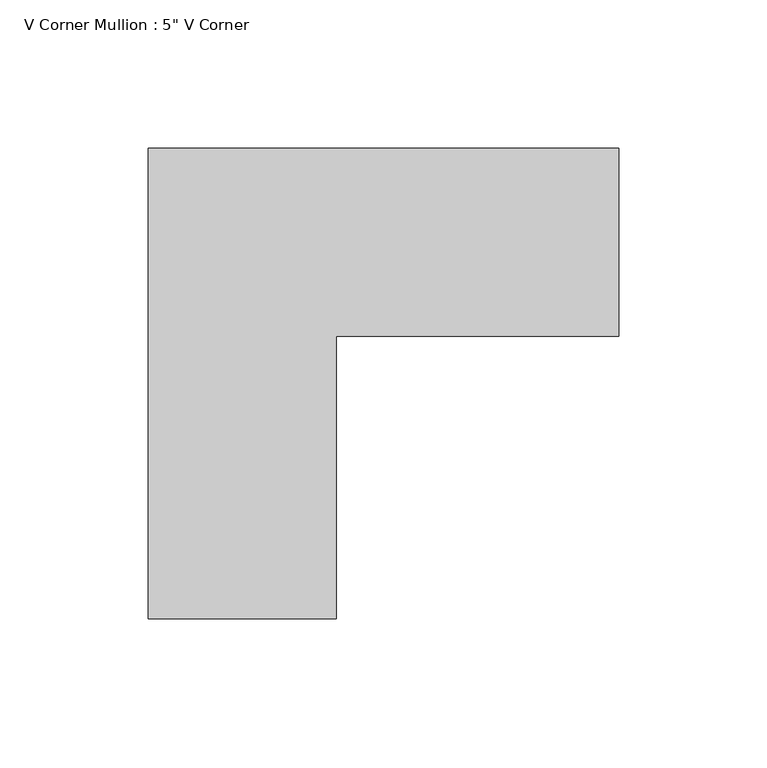
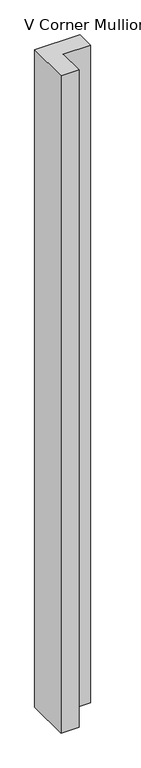
"""IFC4 building model written with IfcOpenShell, lengths in millimetres: member geometry."""

import ifcopenshell
import ifcopenshell.guid

model = None  # the IFC model being written
_history = None  # IfcOwnerHistory: only IFC2X3 demands one
_inside = {}  # id of a spatial element -> (the spatial element, [elements in it])
_under = {}  # id of a project, library or spatial element -> (it, [spatial elements below it])
_declared = {}  # id of a project -> (the project, [libraries it declares])
_typed = {}  # id of a type object -> (the type object, [elements of that type])
_made_of = {}  # id of a material, layer set ... -> (it, [elements and type objects made of it])


def new_model(schema):
    """Start an empty IFC model of exactly this schema.

    Asked for "IFC4X3", IfcOpenShell would pick the latest addendum, in which some entities
    have other attributes; the version numbers below select the first issue.
    IFC2X3 requires an IfcOwnerHistory on every rooted entity: one is made here for all.
    """
    global model, _history
    if schema == "IFC4X3":
        model = ifcopenshell.file(schema_version=(4, 3, 0, 0))
    else:
        model = ifcopenshell.file(schema=schema)
    _inside.clear()
    _under.clear()
    _declared.clear()
    _typed.clear()
    _made_of.clear()
    _history = None
    if model.schema == "IFC2X3":
        org = make("IfcOrganization", Name="unknown")
        user = make(
            "IfcPersonAndOrganization",
            ThePerson=make("IfcPerson", FamilyName="unknown"),
            TheOrganization=org,
        )
        app = make(
            "IfcApplication",
            ApplicationDeveloper=org,
            Version="unknown",
            ApplicationFullName="unknown",
            ApplicationIdentifier="unknown",
        )
        _history = make(
            "IfcOwnerHistory",
            OwningUser=user,
            OwningApplication=app,
            ChangeAction="ADDED",
            CreationDate=0,
        )
    return model


def make(cls, **values):
    """One entity of the class cls with the attributes given. An attribute that is None is left unset."""
    return model.create_entity(
        cls, **{name: value for name, value in values.items() if value is not None}
    )


def rooted(cls, **values):
    """An entity with a GlobalId (a new one), such as an element, a storey or a relation."""
    return make(cls, GlobalId=ifcopenshell.guid.new(), OwnerHistory=_history, **values)


def si_unit(unit_type, name, prefix=None):
    """IfcSIUnit, for example si_unit("LENGTHUNIT", "METRE", prefix="MILLI")."""
    return make("IfcSIUnit", UnitType=unit_type, Prefix=prefix, Name=name)


def assignment(units):
    """IfcUnitAssignment: the units of a project."""
    return None if units is None else make("IfcUnitAssignment", Units=units)


def point(xyz):
    """IfcCartesianPoint."""
    return None if xyz is None else make("IfcCartesianPoint", Coordinates=xyz)


def direction(xyz):
    """IfcDirection."""
    return None if xyz is None else make("IfcDirection", DirectionRatios=xyz)


def frame(location, z_axis=None, x_axis=None):
    """IfcAxis2Placement3D, a coordinate frame: its origin and axes. An axis left out is left unset."""
    return make(
        "IfcAxis2Placement3D",
        Location=point(location),
        Axis=direction(z_axis),
        RefDirection=direction(x_axis),
    )


def origin():
    """The frame at (0, 0, 0) with its axes left unset."""
    return frame((0.0, 0.0, 0.0))


def place(relative_to, where):
    """IfcLocalPlacement: puts the frame where relative to a parent placement (None: the world)."""
    return make(
        "IfcLocalPlacement", PlacementRelTo=relative_to, RelativePlacement=where
    )


def context(
    kind, dimensions, precision=None, world=None, true_north=None, identifier=None
):
    """IfcGeometricRepresentationContext, for example the 3D "Model" context."""
    return make(
        "IfcGeometricRepresentationContext",
        ContextIdentifier=identifier,
        ContextType=kind,
        CoordinateSpaceDimension=dimensions,
        Precision=precision,
        WorldCoordinateSystem=world,
        TrueNorth=true_north,
    )


def project(units=None, contexts=None):
    """IfcProject with its units and contexts."""
    return rooted(
        "IfcProject",
        Name="project",
        RepresentationContexts=contexts,
        UnitsInContext=assignment(units),
    )


def spatial(cls, under=None, at=None, **own):
    """A site, building, storey or space (cls), placed at a placement, below another one or the project."""
    s = rooted(cls, ObjectPlacement=at, **own)
    if under is not None:
        _under.setdefault(under.id(), (under, []))[1].append(s)
    return s


def polyline(points):
    """IfcPolyline through the points."""
    return make("IfcPolyline", Points=[point(p) for p in points])


def outline(outer, holes=None, kind="AREA"):
    """IfcArbitraryClosedProfileDef: a profile drawn as a closed curve; with holes, ...WithVoids."""
    if holes is None:
        return make("IfcArbitraryClosedProfileDef", ProfileType=kind, OuterCurve=outer)
    return make(
        "IfcArbitraryProfileDefWithVoids",
        ProfileType=kind,
        OuterCurve=outer,
        InnerCurves=holes,
    )


def extrude(swept, where, along, depth):
    """IfcExtrudedAreaSolid: the profile swept, set in the frame where, extruded along a direction by depth."""
    return make(
        "IfcExtrudedAreaSolid",
        SweptArea=swept,
        Position=where,
        ExtrudedDirection=direction(along),
        Depth=depth,
    )


def shape(context_of_items, identifier, shape_type, items):
    """IfcShapeRepresentation: the items that make up one representation, for example the "Body"."""
    return make(
        "IfcShapeRepresentation",
        ContextOfItems=context_of_items,
        RepresentationIdentifier=identifier,
        RepresentationType=shape_type,
        Items=items,
    )


def source(mapping_origin, context_of_items, identifier, shape_type, items):
    """IfcRepresentationMap: a shape defined once, which mapped items show again and again."""
    return make(
        "IfcRepresentationMap",
        MappingOrigin=mapping_origin,
        MappedRepresentation=shape(context_of_items, identifier, shape_type, items),
    )


def transform(
    local_origin,
    x_axis=None,
    y_axis=None,
    z_axis=None,
    scale=None,
    scale2=None,
    scale3=None,
    uniform=True,
):
    """IfcCartesianTransformationOperator3D, or its non-uniform kind. x_axis, y_axis, z_axis: its Axis1, 2, 3."""
    if uniform:
        return make(
            "IfcCartesianTransformationOperator3D",
            Axis1=direction(x_axis),
            Axis2=direction(y_axis),
            LocalOrigin=point(local_origin),
            Scale=scale,
            Axis3=direction(z_axis),
        )
    return make(
        "IfcCartesianTransformationOperator3DnonUniform",
        Axis1=direction(x_axis),
        Axis2=direction(y_axis),
        LocalOrigin=point(local_origin),
        Scale=scale,
        Axis3=direction(z_axis),
        Scale2=scale2,
        Scale3=scale3,
    )


def mapped(mapping_source, mapping_target):
    """IfcMappedItem: shows the shape of a source again, moved by a transform."""
    return make(
        "IfcMappedItem", MappingSource=mapping_source, MappingTarget=mapping_target
    )


def made_of(thing, what):
    """Note that an element or type object is made of a material, layer set ...; save() writes the relation."""
    if what is not None:
        _made_of.setdefault(what.id(), (what, []))[1].append(thing)
    return thing


def element(
    cls,
    number,
    at=None,
    inside=None,
    cuts=None,
    type_object=None,
    material=None,
    context=None,
    identifier="Body",
    shape_type=None,
    held_by="IfcProductDefinitionShape",
    body=None,
    shapes=None,
    **own,
):
    """One element of the class cls, such as IfcWall. Its Tag is "e" and its number.

    at: its placement. inside: the storey or other place that contains it. cuts: it is an
    opening in that element (IfcRelVoidsElement). A single representation is given by context,
    identifier, shape_type and body (its items); several are given by shapes. held_by: the class
    of the entity that holds the representations. save() writes the other relations.
    """
    e = rooted(cls, Tag="e%d" % number, ObjectPlacement=at, **own)
    if body is not None:
        shapes = [shape(context, identifier, shape_type, body)]
    if shapes is not None:
        e.Representation = make(held_by, Representations=shapes)
    if inside is not None:
        _inside.setdefault(inside.id(), (inside, []))[1].append(e)
    if cuts is not None:
        rooted(
            "IfcRelVoidsElement", RelatingBuildingElement=cuts, RelatedOpeningElement=e
        )
    if type_object is not None:
        _typed.setdefault(type_object.id(), (type_object, []))[1].append(e)
    return made_of(e, material)


def aggregate(whole, parts):
    """IfcRelAggregates: a whole, such as a stair, and the parts it consists of."""
    return rooted("IfcRelAggregates", RelatingObject=whole, RelatedObjects=parts)


def save(model, path):
    """Write the relations noted so far, then the file.

    IfcRelAggregates (storeys below a building ...), IfcRelContainedInSpatialStructure (elements
    in a storey), IfcRelDefinesByType, IfcRelAssociatesMaterial and IfcRelDeclares: one each for
    every whole, place, type object, material and project.
    """
    for whole, parts in _under.values():
        aggregate(whole, parts)
    for where, things in _inside.values():
        rooted(
            "IfcRelContainedInSpatialStructure",
            RelatedElements=things,
            RelatingStructure=where,
        )
    for kind, things in _typed.values():
        rooted("IfcRelDefinesByType", RelatedObjects=things, RelatingType=kind)
    for what, things in _made_of.values():
        rooted("IfcRelAssociatesMaterial", RelatedObjects=things, RelatingMaterial=what)
    for by, libraries in _declared.values():
        rooted("IfcRelDeclares", RelatingContext=by, RelatedDefinitions=libraries)
    model.write(path)


def member_ea83204a(model_context):
    return source(origin(), model_context, "Body", "SweptSolid", [
        extrude(outline(polyline([(63.5, 31.75), (-31.75, 31.75), (-31.75, -63.5), (-95.25, -63.5), (-95.25, 95.25), (63.5, 95.25), (63.5, 31.75)])), frame((0.0, 0.0, -2438.4), z_axis=(0.0, 0.0, 1.0), x_axis=(1.0, 0.0, 0.0)), (0.0, 0.0, 1.0), 2438.4),
    ])


if __name__ == "__main__":
    model = new_model("IFC4")
    model_context = context("Model", 3, world=origin())
    ifc_project = project(units=[si_unit("LENGTHUNIT", "METRE", prefix="MILLI")], contexts=[model_context])
    site = spatial("IfcSite", under=ifc_project)
    building = spatial("IfcBuilding", under=site)
    placement = place(None, origin())
    member_shape = member_ea83204a(model_context)
    element("IfcMember", 1, ObjectType="V Corner Mullion : 5\" V Corner", at=placement, inside=building, context=model_context, shape_type="MappedRepresentation", body=[
        mapped(member_shape, transform((0.0, 0.0, 0.0), x_axis=(1.0, 0.0, 0.0), y_axis=(0.0, 1.0, 0.0), z_axis=(0.0, 0.0, 1.0))),
    ])
    save(model, "model.ifc")

# Revit data of these elements
# Type "V Corner Mullion : 5\" V Corner"
#   built-in parameter 1007355 = 0.416667 (stored number, unit not read)
#   built-in parameter 1007354 = 0.416667 (stored number, unit not read)
#   built-in parameter 1007304 = 0.208333 (stored number, unit not read)
